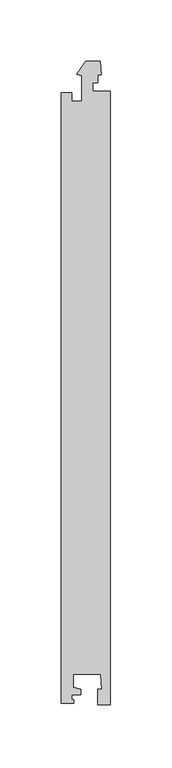
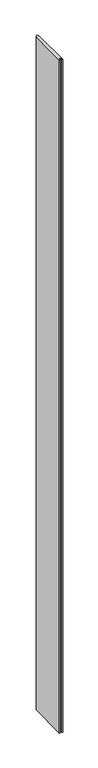
"""IFC4 building model written with IfcOpenShell, lengths in millimetres: proxy geometry, Generic Models 5:Generic Models 5:321804:Generic Models 5:321804 : Generic Models 5:Generic Models 5:321804:36 : Generic Models 5:Generic Models 5:321804:Generic Models 5:321804 : Generic Models 5:Generic Models 5:321804:300761."""

from ifc_helpers import new_model, si_unit, frame, origin, place, context, project, spatial, polyline, outline, extrude, source, transform, mapped, element, save


def generic_models_1dd85ba2(model_context):
    return source(origin(), model_context, "Body", "SweptSolid", [
        extrude(outline(polyline([(667625.2338797, -491410.833465), (667631.7338797, -491412.5751348), (667631.7338797, -491417.0251348), (667624.2338797, -491417.0251348), (667624.2338797, -491420.9751348), (667625.7338797, -491420.9751348), (667625.7338797, -491423.9751348), (667615.7338797, -491423.9751348), (667615.7338797, -490926.4751348), (667624.2338797, -490926.4751348), (667624.2338797, -490933.4251348), (667632.2338797, -490933.4251348), (667632.2338797, -490912.7091094), (667628.3059983, -490911.6566367), (667635.4133634, -490900.9751348), (667647.2715044, -490900.9751348), (667648.2338797, -490911.9751348), (667645.5338797, -490911.9751348), (667645.5338797, -490918.6001348), (667641.2338797, -490918.6001348), (667641.2338797, -490925.2251348), (667655.7338797, -490925.2251348), (667655.7338797, -491425.2251348), (667645.5338797, -491425.2251348), (667645.5338797, -491412.4751348), (667648.779534, -491412.4751348), (667647.72967, -491400.4751348), (667625.2338797, -491400.4751348), (667625.2338797, -491410.833465)])), frame((0.0, 0.0, -5.8417589), z_axis=(0.0, 0.0, 1.0), x_axis=(1.0, 0.0, 0.0)), (0.0, 0.0, 1.0), 8779.7126309),
    ])


if __name__ == "__main__":
    model = new_model("IFC4")
    model_context = context("Model", 3, world=origin())
    ifc_project = project(units=[si_unit("LENGTHUNIT", "METRE", prefix="MILLI")], contexts=[model_context])
    site = spatial("IfcSite", under=ifc_project)
    building = spatial("IfcBuilding", under=site)
    placement = place(None, origin())
    generic_models_shape = generic_models_1dd85ba2(model_context)
    element("IfcBuildingElementProxy", 1, Name="Generic Models 5:Generic Models 5:321804:Generic Models 5:321804 : Generic Models 5:Generic Models 5:321804:36 : Generic Models 5:Generic Models 5:321804:Generic Models 5:321804 : Generic Models 5:Generic Models 5:321804:300761", ObjectType="Generic Models 5:Generic Models 5:321804:Generic Models 5:321804 : Generic Models 5:Generic Models 5:321804:36 : Generic Models 5:Generic Models 5:321804:Generic Models 5:321804 : Generic Models 5:Generic Models 5:321804:300761", at=placement, inside=building, context=model_context, shape_type="MappedRepresentation", body=[
        mapped(generic_models_shape, transform((0.0, 0.0, 0.0), x_axis=(1.0, 0.0, 0.0), y_axis=(0.0, 1.0, 0.0), z_axis=(0.0, 0.0, 1.0))),
    ])
    save(model, "model.ifc")

# Revit data of these elements
# Type "Generic Models 5:Generic Models 5:321804:Generic Models 5:321804 : Generic Models 5:Generic Models 5:321804:36 : Generic Models 5:Generic Models 5:321804:Generic Models 5:321804 : Generic Models 5:Generic Models 5:321804:300761"
#   NameOverride = "Generic Models 5:Generic Models 5:321804:Generic Models 5:321804 : Generic Models 5:Generic Models 5:321804:300761"
#   ObjectTypeOverride = "Generic Models 5:321804 : Generic Models 5:Generic Models 5:321804"
#   Reference = "Generic Models 5"
#   Tag = "300761"
# Element 1 (IfcBuildingElementProxy, "Generic Models 5:Generic Models 5:321804:Generic Models 5:321804 : Generic Models 5:Generic Models 5:321804:36 : Generic Models 5:Generic Models 5:321804:Generic Models 5:321804 : Generic Models 5:Generic Models 5:321804:300761")
#   Materials on its faces: "POLYCARBONATE PANEL - ARCOPLUS 547"
# Materials
#   "POLYCARBONATE PANEL - ARCOPLUS 547": class "Unassigned", colour RGB 202 225 249, transparency 0.45, Cost = 0
